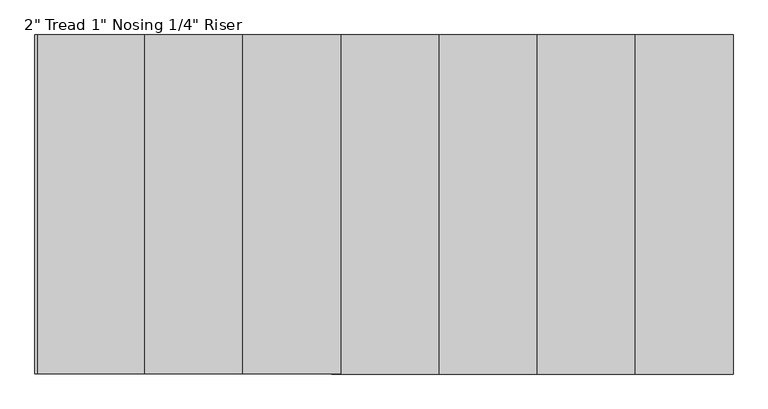
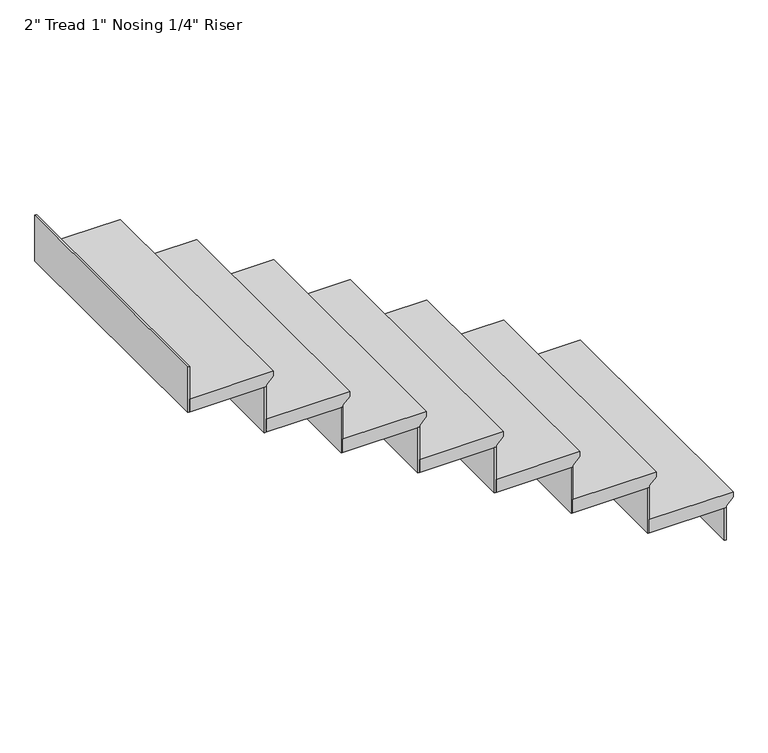
"""IFC4 building model written with IfcOpenShell, lengths in millimetres: stair flight geometry."""

import ifcopenshell
import ifcopenshell.guid

model = None  # the IFC model being written
_history = None  # IfcOwnerHistory: only IFC2X3 demands one
_inside = {}  # id of a spatial element -> (the spatial element, [elements in it])
_under = {}  # id of a project, library or spatial element -> (it, [spatial elements below it])
_declared = {}  # id of a project -> (the project, [libraries it declares])
_typed = {}  # id of a type object -> (the type object, [elements of that type])
_made_of = {}  # id of a material, layer set ... -> (it, [elements and type objects made of it])


def new_model(schema):
    """Start an empty IFC model of exactly this schema.

    Asked for "IFC4X3", IfcOpenShell would pick the latest addendum, in which some entities
    have other attributes; the version numbers below select the first issue.
    IFC2X3 requires an IfcOwnerHistory on every rooted entity: one is made here for all.
    """
    global model, _history
    if schema == "IFC4X3":
        model = ifcopenshell.file(schema_version=(4, 3, 0, 0))
    else:
        model = ifcopenshell.file(schema=schema)
    _inside.clear()
    _under.clear()
    _declared.clear()
    _typed.clear()
    _made_of.clear()
    _history = None
    if model.schema == "IFC2X3":
        org = make("IfcOrganization", Name="unknown")
        user = make(
            "IfcPersonAndOrganization",
            ThePerson=make("IfcPerson", FamilyName="unknown"),
            TheOrganization=org,
        )
        app = make(
            "IfcApplication",
            ApplicationDeveloper=org,
            Version="unknown",
            ApplicationFullName="unknown",
            ApplicationIdentifier="unknown",
        )
        _history = make(
            "IfcOwnerHistory",
            OwningUser=user,
            OwningApplication=app,
            ChangeAction="ADDED",
            CreationDate=0,
        )
    return model


def make(cls, **values):
    """One entity of the class cls with the attributes given. An attribute that is None is left unset."""
    return model.create_entity(
        cls, **{name: value for name, value in values.items() if value is not None}
    )


def rooted(cls, **values):
    """An entity with a GlobalId (a new one), such as an element, a storey or a relation."""
    return make(cls, GlobalId=ifcopenshell.guid.new(), OwnerHistory=_history, **values)


def si_unit(unit_type, name, prefix=None):
    """IfcSIUnit, for example si_unit("LENGTHUNIT", "METRE", prefix="MILLI")."""
    return make("IfcSIUnit", UnitType=unit_type, Prefix=prefix, Name=name)


def assignment(units):
    """IfcUnitAssignment: the units of a project."""
    return None if units is None else make("IfcUnitAssignment", Units=units)


def point(xyz):
    """IfcCartesianPoint."""
    return None if xyz is None else make("IfcCartesianPoint", Coordinates=xyz)


def direction(xyz):
    """IfcDirection."""
    return None if xyz is None else make("IfcDirection", DirectionRatios=xyz)


def frame(location, z_axis=None, x_axis=None):
    """IfcAxis2Placement3D, a coordinate frame: its origin and axes. An axis left out is left unset."""
    return make(
        "IfcAxis2Placement3D",
        Location=point(location),
        Axis=direction(z_axis),
        RefDirection=direction(x_axis),
    )


def origin():
    """The frame at (0, 0, 0) with its axes left unset."""
    return frame((0.0, 0.0, 0.0))


def place(relative_to, where):
    """IfcLocalPlacement: puts the frame where relative to a parent placement (None: the world)."""
    return make(
        "IfcLocalPlacement", PlacementRelTo=relative_to, RelativePlacement=where
    )


def context(
    kind, dimensions, precision=None, world=None, true_north=None, identifier=None
):
    """IfcGeometricRepresentationContext, for example the 3D "Model" context."""
    return make(
        "IfcGeometricRepresentationContext",
        ContextIdentifier=identifier,
        ContextType=kind,
        CoordinateSpaceDimension=dimensions,
        Precision=precision,
        WorldCoordinateSystem=world,
        TrueNorth=true_north,
    )


def project(units=None, contexts=None):
    """IfcProject with its units and contexts."""
    return rooted(
        "IfcProject",
        Name="project",
        RepresentationContexts=contexts,
        UnitsInContext=assignment(units),
    )


def spatial(cls, under=None, at=None, **own):
    """A site, building, storey or space (cls), placed at a placement, below another one or the project."""
    s = rooted(cls, ObjectPlacement=at, **own)
    if under is not None:
        _under.setdefault(under.id(), (under, []))[1].append(s)
    return s


def faces_of(points, faces, orient=None, outer=None):
    """IfcFace entities. A face is a list of loops; a loop is a list of indices into points, from 0.

    orient and outer hold one flag for each loop. By default every Orientation is true, the
    first loop of a face is its IfcFaceOuterBound and the others are IfcFaceBound.
    """
    made = []
    for i, loops in enumerate(faces):
        bounds = []
        for j, loop in enumerate(loops):
            is_outer = j == 0 if outer is None else outer[i][j]
            bounds.append(
                make(
                    "IfcFaceOuterBound" if is_outer else "IfcFaceBound",
                    Bound=make("IfcPolyLoop", Polygon=[points[k] for k in loop]),
                    Orientation=True if orient is None else orient[i][j],
                )
            )
        made.append(make("IfcFace", Bounds=bounds))
    return made


def faceted_brep(points, faces, orient=None, outer=None, voids=None):
    """IfcFacetedBrep: a solid bounded by flat faces; with voids (closed shells), ...WithVoids."""
    shared = [point(p) for p in points]
    hull = make("IfcClosedShell", CfsFaces=faces_of(shared, faces, orient, outer))
    if voids is None:
        return make("IfcFacetedBrep", Outer=hull)
    return make(
        "IfcFacetedBrepWithVoids",
        Outer=hull,
        Voids=[
            make(cls, CfsFaces=faces_of(shared, fs, o, b)) for cls, fs, o, b in voids
        ],
    )


def shape(context_of_items, identifier, shape_type, items):
    """IfcShapeRepresentation: the items that make up one representation, for example the "Body"."""
    return make(
        "IfcShapeRepresentation",
        ContextOfItems=context_of_items,
        RepresentationIdentifier=identifier,
        RepresentationType=shape_type,
        Items=items,
    )


def source(mapping_origin, context_of_items, identifier, shape_type, items):
    """IfcRepresentationMap: a shape defined once, which mapped items show again and again."""
    return make(
        "IfcRepresentationMap",
        MappingOrigin=mapping_origin,
        MappedRepresentation=shape(context_of_items, identifier, shape_type, items),
    )


def transform(
    local_origin,
    x_axis=None,
    y_axis=None,
    z_axis=None,
    scale=None,
    scale2=None,
    scale3=None,
    uniform=True,
):
    """IfcCartesianTransformationOperator3D, or its non-uniform kind. x_axis, y_axis, z_axis: its Axis1, 2, 3."""
    if uniform:
        return make(
            "IfcCartesianTransformationOperator3D",
            Axis1=direction(x_axis),
            Axis2=direction(y_axis),
            LocalOrigin=point(local_origin),
            Scale=scale,
            Axis3=direction(z_axis),
        )
    return make(
        "IfcCartesianTransformationOperator3DnonUniform",
        Axis1=direction(x_axis),
        Axis2=direction(y_axis),
        LocalOrigin=point(local_origin),
        Scale=scale,
        Axis3=direction(z_axis),
        Scale2=scale2,
        Scale3=scale3,
    )


def mapped(mapping_source, mapping_target):
    """IfcMappedItem: shows the shape of a source again, moved by a transform."""
    return make(
        "IfcMappedItem", MappingSource=mapping_source, MappingTarget=mapping_target
    )


def made_of(thing, what):
    """Note that an element or type object is made of a material, layer set ...; save() writes the relation."""
    if what is not None:
        _made_of.setdefault(what.id(), (what, []))[1].append(thing)
    return thing


def element(
    cls,
    number,
    at=None,
    inside=None,
    cuts=None,
    type_object=None,
    material=None,
    context=None,
    identifier="Body",
    shape_type=None,
    held_by="IfcProductDefinitionShape",
    body=None,
    shapes=None,
    **own,
):
    """One element of the class cls, such as IfcWall. Its Tag is "e" and its number.

    at: its placement. inside: the storey or other place that contains it. cuts: it is an
    opening in that element (IfcRelVoidsElement). A single representation is given by context,
    identifier, shape_type and body (its items); several are given by shapes. held_by: the class
    of the entity that holds the representations. save() writes the other relations.
    """
    e = rooted(cls, Tag="e%d" % number, ObjectPlacement=at, **own)
    if body is not None:
        shapes = [shape(context, identifier, shape_type, body)]
    if shapes is not None:
        e.Representation = make(held_by, Representations=shapes)
    if inside is not None:
        _inside.setdefault(inside.id(), (inside, []))[1].append(e)
    if cuts is not None:
        rooted(
            "IfcRelVoidsElement", RelatingBuildingElement=cuts, RelatedOpeningElement=e
        )
    if type_object is not None:
        _typed.setdefault(type_object.id(), (type_object, []))[1].append(e)
    return made_of(e, material)


def aggregate(whole, parts):
    """IfcRelAggregates: a whole, such as a stair, and the parts it consists of."""
    return rooted("IfcRelAggregates", RelatingObject=whole, RelatedObjects=parts)


def save(model, path):
    """Write the relations noted so far, then the file.

    IfcRelAggregates (storeys below a building ...), IfcRelContainedInSpatialStructure (elements
    in a storey), IfcRelDefinesByType, IfcRelAssociatesMaterial and IfcRelDeclares: one each for
    every whole, place, type object, material and project.
    """
    for whole, parts in _under.values():
        aggregate(whole, parts)
    for where, things in _inside.values():
        rooted(
            "IfcRelContainedInSpatialStructure",
            RelatedElements=things,
            RelatingStructure=where,
        )
    for kind, things in _typed.values():
        rooted("IfcRelDefinesByType", RelatedObjects=things, RelatingType=kind)
    for what, things in _made_of.values():
        rooted("IfcRelAssociatesMaterial", RelatedObjects=things, RelatingMaterial=what)
    for by, libraries in _declared.values():
        rooted("IfcRelDeclares", RelatingContext=by, RelatedDefinitions=libraries)
    model.write(path)


def stair_flight_8c0a896d(model_context):
    return source(origin(), model_context, "Body", "Brep", [
        faceted_brep([(26763.6590778, 27767.6156612, 266551.56875), (26763.6590778, 27767.6156612, 266570.61875), (26763.6590778, 26802.4156612, 266570.61875), (26763.6590778, 26802.4156612, 266551.56875), (26738.2590778, 27767.6156612, 266526.16875), (26738.2590778, 26802.4156612, 266526.16875), (26458.8590778, 27767.6156612, 266570.61875), (26458.8590778, 26802.4156612, 266570.61875), (26738.2590778, 26802.4156612, 266519.81875), (26458.8590778, 26802.4156612, 266519.81875), (26458.8590778, 27767.6156612, 266519.81875), (26738.2590778, 27767.6156612, 266519.81875)], [[[0, 1, 2, 3]], [[4, 0, 3, 5]], [[2, 1, 6, 7]], [[8, 9, 10, 11]], [[2, 7, 9, 8, 5, 3]], [[8, 11, 4, 5]], [[6, 1, 0, 4, 11, 10]], [[7, 6, 10, 9]]]),
        faceted_brep([(26738.2590778, 27767.6156612, 266519.81875), (26738.2590778, 27767.6156612, 266395.2), (26731.9090778, 27767.6156612, 266395.2), (26731.9090778, 27767.6156612, 266519.81875), (26738.2590778, 26802.4156612, 266519.81875), (26731.9090778, 26802.4156612, 266519.81875), (26731.9090778, 26802.4156612, 266395.2), (26738.2590778, 26802.4156612, 266395.2)], [[[0, 1, 2, 3]], [[4, 5, 6, 7]], [[1, 0, 4, 7]], [[2, 1, 7, 6]], [[3, 2, 6, 5]], [[0, 3, 5, 4]]]),
        faceted_brep([(26458.8590778, 27767.6156612, 266695.2375), (26458.8590778, 27767.6156612, 266519.81875), (26452.5090778, 27767.6156612, 266519.81875), (26452.5090778, 27767.6156612, 266695.2375), (26458.8590778, 26802.4156612, 266695.2375), (26452.5090778, 26802.4156612, 266695.2375), (26452.5090778, 26802.4156612, 266519.81875), (26458.8590778, 26802.4156612, 266519.81875)], [[[0, 1, 2, 3]], [[4, 5, 6, 7]], [[1, 0, 4, 7]], [[2, 1, 7, 6]], [[3, 2, 6, 5]], [[0, 3, 5, 4]]]),
        faceted_brep([(26484.2590778, 26802.4156612, 266746.0375), (26484.2590778, 27767.6156612, 266746.0375), (26179.4590778, 27767.6156612, 266746.0375), (26179.4590778, 26802.4156612, 266746.0375), (26458.8590778, 26802.4156612, 266695.2375), (26179.4590778, 26802.4156612, 266695.2375), (26179.4590778, 27767.6156612, 266695.2375), (26458.8590778, 27767.6156612, 266695.2375), (26458.8590778, 26802.4156612, 266701.5875), (26484.2590778, 26802.4156612, 266726.9875), (26458.8590778, 27767.6156612, 266701.5875), (26484.2590778, 27767.6156612, 266726.9875)], [[[0, 1, 2, 3]], [[4, 5, 6, 7]], [[0, 3, 5, 4, 8, 9]], [[4, 7, 10, 8]], [[2, 1, 11, 10, 7, 6]], [[3, 2, 6, 5]], [[11, 1, 0, 9]], [[10, 11, 9, 8]]]),
        faceted_brep([(26179.4590778, 27767.6156612, 266870.65625), (26179.4590778, 27767.6156612, 266695.2375), (26173.1090778, 27767.6156612, 266695.2375), (26173.1090778, 27767.6156612, 266870.65625), (26179.4590778, 26802.4156612, 266870.65625), (26173.1090778, 26802.4156612, 266870.65625), (26173.1090778, 26802.4156612, 266695.2375), (26179.4590778, 26802.4156612, 266695.2375)], [[[0, 1, 2, 3]], [[4, 5, 6, 7]], [[1, 0, 4, 7]], [[2, 1, 7, 6]], [[3, 2, 6, 5]], [[0, 3, 5, 4]]]),
        faceted_brep([(26204.8590778, 26802.4156612, 266921.45625), (26204.8590778, 27767.6156612, 266921.45625), (25900.0590778, 27767.6156612, 266921.45625), (25900.0590778, 26802.4156612, 266921.45625), (26179.4590778, 26802.4156612, 266870.65625), (25900.0590778, 26802.4156612, 266870.65625), (25900.0590778, 27767.6156612, 266870.65625), (26179.4590778, 27767.6156612, 266870.65625), (26179.4590778, 26802.4156612, 266877.00625), (26204.8590778, 26802.4156612, 266902.40625), (26179.4590778, 27767.6156612, 266877.00625), (26204.8590778, 27767.6156612, 266902.40625)], [[[0, 1, 2, 3]], [[4, 5, 6, 7]], [[0, 3, 5, 4, 8, 9]], [[4, 7, 10, 8]], [[2, 1, 11, 10, 7, 6]], [[3, 2, 6, 5]], [[11, 1, 0, 9]], [[10, 11, 9, 8]]]),
        faceted_brep([(25900.0590778, 27767.6156612, 267046.075), (25900.0590778, 27767.6156612, 266870.65625), (25893.7090778, 27767.6156612, 266870.65625), (25893.7090778, 27767.6156612, 267046.075), (25900.0590778, 26802.4156612, 267046.075), (25893.7090778, 26802.4156612, 267046.075), (25893.7090778, 26802.4156612, 266870.65625), (25900.0590778, 26802.4156612, 266870.65625)], [[[0, 1, 2, 3]], [[4, 5, 6, 7]], [[1, 0, 4, 7]], [[2, 1, 7, 6]], [[3, 2, 6, 5]], [[0, 3, 5, 4]]]),
        faceted_brep([(25925.4590778, 26802.4156612, 267096.875), (25925.4590778, 27767.6156612, 267096.875), (25620.6590778, 27767.6156612, 267096.875), (25620.6590778, 26802.4156612, 267096.875), (25900.0590778, 26802.4156612, 267046.075), (25620.6590778, 26802.4156612, 267046.075), (25620.6590778, 27767.6156612, 267046.075), (25900.0590778, 27767.6156612, 267046.075), (25900.0590778, 26802.4156612, 267052.425), (25925.4590778, 26802.4156612, 267077.825), (25900.0590778, 27767.6156612, 267052.425), (25925.4590778, 27767.6156612, 267077.825)], [[[0, 1, 2, 3]], [[4, 5, 6, 7]], [[0, 3, 5, 4, 8, 9]], [[4, 7, 10, 8]], [[2, 1, 11, 10, 7, 6]], [[3, 2, 6, 5]], [[11, 1, 0, 9]], [[10, 11, 9, 8]]]),
        faceted_brep([(25620.6590778, 27767.6156612, 267221.49375), (25620.6590778, 27767.6156612, 267046.075), (25614.3090778, 27767.6156612, 267046.075), (25614.3090778, 27767.6156612, 267221.49375), (25620.6590778, 26802.4156612, 267221.49375), (25614.3090778, 26802.4156612, 267221.49375), (25614.3090778, 26802.4156612, 267046.075), (25620.6590778, 26802.4156612, 267046.075)], [[[0, 1, 2, 3]], [[4, 5, 6, 7]], [[1, 0, 4, 7]], [[2, 1, 7, 6]], [[3, 2, 6, 5]], [[0, 3, 5, 4]]]),
        faceted_brep([(25646.0590778, 26802.4156612, 267272.29375), (25646.0590778, 27767.6156612, 267272.29375), (25341.2590778, 27767.6156612, 267272.29375), (25341.2590778, 26802.4156612, 267272.29375), (25620.6590778, 26802.4156612, 267221.49375), (25341.2590778, 26802.4156612, 267221.49375), (25341.2590778, 27767.6156612, 267221.49375), (25620.6590778, 27767.6156612, 267221.49375), (25620.6590778, 26802.4156612, 267227.84375), (25646.0590778, 26802.4156612, 267253.24375), (25620.6590778, 27767.6156612, 267227.84375), (25646.0590778, 27767.6156612, 267253.24375)], [[[0, 1, 2, 3]], [[4, 5, 6, 7]], [[0, 3, 5, 4, 8, 9]], [[4, 7, 10, 8]], [[2, 1, 11, 10, 7, 6]], [[3, 2, 6, 5]], [[11, 1, 0, 9]], [[10, 11, 9, 8]]]),
        faceted_brep([(25341.2590778, 27767.6156612, 267396.9125), (25341.2590778, 27767.6156612, 267221.49375), (25334.9090778, 27767.6156612, 267221.49375), (25334.9090778, 27767.6156612, 267396.9125), (25341.2590778, 26802.4156612, 267396.9125), (25334.9090778, 26802.4156612, 267396.9125), (25334.9090778, 26802.4156612, 267221.49375), (25341.2590778, 26802.4156612, 267221.49375)], [[[0, 1, 2, 3]], [[4, 5, 6, 7]], [[1, 0, 4, 7]], [[2, 1, 7, 6]], [[3, 2, 6, 5]], [[0, 3, 5, 4]]]),
        faceted_brep([(25366.6590778, 26802.4156612, 267447.7125), (25366.6590778, 27767.6156612, 267447.7125), (25061.8590778, 27767.6156612, 267447.7125), (25061.8590778, 26802.4156612, 267447.7125), (25341.2590778, 26802.4156612, 267396.9125), (25061.8590778, 26802.4156612, 267396.9125), (25061.8590778, 27767.6156612, 267396.9125), (25341.2590778, 27767.6156612, 267396.9125), (25341.2590778, 26802.4156612, 267403.2625), (25366.6590778, 26802.4156612, 267428.6625), (25341.2590778, 27767.6156612, 267403.2625), (25366.6590778, 27767.6156612, 267428.6625)], [[[0, 1, 2, 3]], [[4, 5, 6, 7]], [[0, 3, 5, 4, 8, 9]], [[4, 7, 10, 8]], [[2, 1, 11, 10, 7, 6]], [[3, 2, 6, 5]], [[11, 1, 0, 9]], [[10, 11, 9, 8]]]),
        faceted_brep([(24782.4590778, 27767.6156612, 267747.75), (24782.4590778, 27767.6156612, 267572.33125), (24776.1090778, 27767.6156612, 267572.33125), (24776.1090778, 27767.6156612, 267747.75), (24782.4590778, 26802.4156612, 267747.75), (24776.1090778, 26802.4156612, 267747.75), (24776.1090778, 26802.4156612, 267572.33125), (24782.4590778, 26802.4156612, 267572.33125)], [[[0, 1, 2, 3]], [[4, 5, 6, 7]], [[1, 0, 4, 7]], [[2, 1, 7, 6]], [[3, 2, 6, 5]], [[0, 3, 5, 4]]]),
        faceted_brep([(25061.8590778, 27767.6156612, 267572.33125), (25061.8590778, 27767.6156612, 267396.9125), (25055.5090778, 27767.6156612, 267396.9125), (25055.5090778, 27767.6156612, 267572.33125), (25061.8590778, 26802.4156612, 267572.33125), (25055.5090778, 26802.4156612, 267572.33125), (25055.5090778, 26802.4156612, 267396.9125), (25061.8590778, 26802.4156612, 267396.9125)], [[[0, 1, 2, 3]], [[4, 5, 6, 7]], [[1, 0, 4, 7]], [[2, 1, 7, 6]], [[3, 2, 6, 5]], [[0, 3, 5, 4]]]),
        faceted_brep([(25087.2590778, 26802.4156612, 267623.13125), (25087.2590778, 27767.6156612, 267623.13125), (24807.8590778, 27767.6156612, 267623.13125), (24782.4590778, 27767.6156612, 267623.13125), (24782.4590778, 26802.4156612, 267623.13125), (25061.8590778, 26802.4156612, 267572.33125), (24782.4590778, 26802.4156612, 267572.33125), (24782.4590778, 27767.6156612, 267572.33125), (24807.8590778, 27767.6156612, 267572.33125), (25061.8590778, 27767.6156612, 267572.33125), (25061.8590778, 26802.4156612, 267578.68125), (25087.2590778, 26802.4156612, 267604.08125), (25061.8590778, 27767.6156612, 267578.68125), (25087.2590778, 27767.6156612, 267604.08125)], [[[0, 1, 2, 3, 4]], [[5, 6, 7, 8, 9]], [[0, 4, 6, 5, 10, 11]], [[5, 9, 12, 10]], [[2, 1, 13, 12, 9, 8]], [[4, 3, 7, 6]], [[13, 1, 0, 11]], [[12, 13, 11, 10]], [[3, 2, 8, 7]]]),
    ])


if __name__ == "__main__":
    model = new_model("IFC4")
    model_context = context("Model", 3, world=origin())
    ifc_project = project(units=[si_unit("LENGTHUNIT", "METRE", prefix="MILLI")], contexts=[model_context])
    site = spatial("IfcSite", under=ifc_project)
    building = spatial("IfcBuilding", under=site)
    placement = place(None, origin())
    stair_flight_shape = stair_flight_8c0a896d(model_context)
    element("IfcStairFlight", 1, ObjectType="2\" Tread 1\" Nosing 1/4\" Riser", at=placement, inside=building, context=model_context, shape_type="MappedRepresentation", body=[
        mapped(stair_flight_shape, transform((0.0, 0.0, 0.0), x_axis=(1.0, 0.0, 0.0), y_axis=(0.0, 1.0, 0.0), z_axis=(0.0, 0.0, 1.0))),
    ])
    save(model, "model.ifc")

# Revit data of these elements
# Element 1 (IfcStairFlight, "2\" Tread 1\" Nosing 1/4\" Riser")
#   Materials on its faces: "SLOTTED WOOD FENCE (THERMALLY MODIFIED WOOD: ARBOR WOOD)\n(EXTERIOR STAIN : PENOFIN VERDE EXT. STAIN - COLOR: CEDAR)"
# Materials
#   "SLOTTED WOOD FENCE (THERMALLY MODIFIED WOOD: ARBOR WOOD)\n(EXTERIOR STAIN : PENOFIN VERDE EXT. STAIN - COLOR: CEDAR)": class "Wood", colour RGB 164 134 123, transparency 0, Description = "Pinus Echinata", Cost = 0
